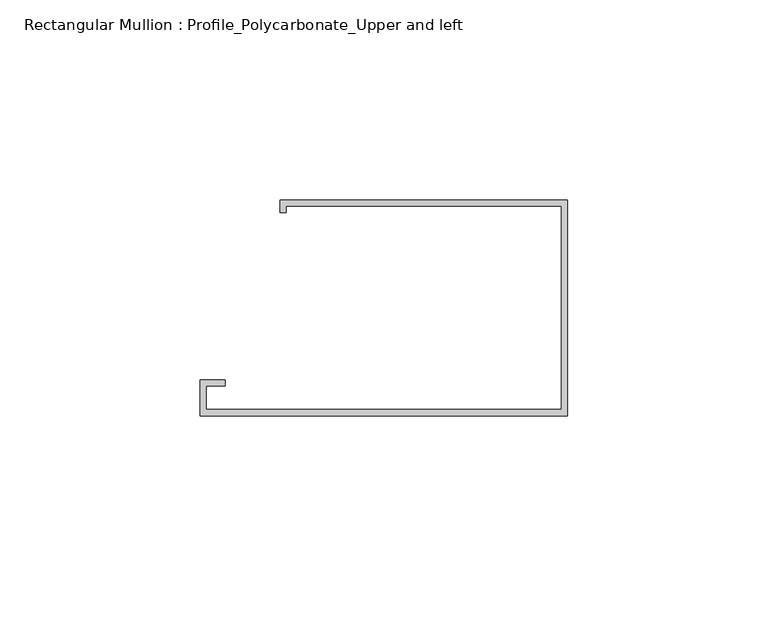
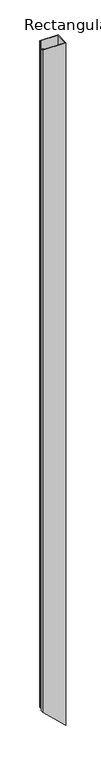
"""IFC4 building model written with IfcOpenShell, lengths in millimetres: member geometry, Rectangular Mullion : Profile_Polycarbonate_Upper and left."""

from ifc_helpers import new_model, si_unit, origin, place, context, project, spatial, faceted_brep, source, transform, mapped, element, save


def rectangular_mullion_profile_polycarbonate_upper_and_left_c928ab11(model_context):
    return source(origin(), model_context, "Body", "Brep", [
        faceted_brep([(0.0, -28.984575, 0.0), (0.0, 25.015825, 0.0), (-71.9836, 25.015825, 0.0), (-71.9836, 21.840825, 0.0), (-70.3961, 21.840825, 0.0), (-70.3961, 23.428325, 0.0), (-1.5875, 23.428325, 0.0), (-1.5875, -27.397075, 0.0), (-90.4113, -27.397075, 0.0), (-90.4113, -21.580475, 0.0), (-85.6488, -21.580475, 0.0), (-85.6488, -19.992975, 0.0), (-91.9988, -19.992975, 0.0), (-91.9988, -28.984575, 0.0), (0.0, -28.984575, -2875.2880888), (0.0, 25.015825, -2875.2880888), (-71.9836, 25.015825, -2806.2413468), (-71.9836, 21.840825, -2806.2413468), (-70.3961, 21.840825, -2807.7640784), (-70.3961, 23.428325, -2807.7640784), (-1.5875, 23.428325, -2873.7653572), (-1.5875, -27.397075, -2873.7653572), (-90.4113, -27.397075, -2788.5654783), (-90.4113, -21.580475, -2788.5654783), (-85.6488, -21.580475, -2793.1336732), (-85.6488, -19.992975, -2793.1336732), (-91.9988, -19.992975, -2787.0427467), (-91.9988, -28.984575, -2787.0427467)], [[[0, 1, 2, 3, 4, 5, 6, 7, 8, 9, 10, 11, 12, 13]], [[1, 0, 14, 15]], [[2, 1, 15, 16]], [[3, 2, 16, 17]], [[4, 3, 17, 18]], [[5, 4, 18, 19]], [[6, 5, 19, 20]], [[7, 6, 20, 21]], [[8, 7, 21, 22]], [[9, 8, 22, 23]], [[10, 9, 23, 24]], [[11, 10, 24, 25]], [[12, 11, 25, 26]], [[13, 12, 26, 27]], [[0, 13, 27, 14]], [[14, 27, 26, 25, 24, 23, 22, 21, 20, 19, 18, 17, 16, 15]]]),
    ])


if __name__ == "__main__":
    model = new_model("IFC4")
    model_context = context("Model", 3, world=origin())
    ifc_project = project(units=[si_unit("LENGTHUNIT", "METRE", prefix="MILLI")], contexts=[model_context])
    site = spatial("IfcSite", under=ifc_project)
    building = spatial("IfcBuilding", under=site)
    placement = place(None, origin())
    rectangular_mullion_profile_polycarbonate_upper_and_left_shape = rectangular_mullion_profile_polycarbonate_upper_and_left_c928ab11(model_context)
    element("IfcMember", 1, ObjectType="Rectangular Mullion : Profile_Polycarbonate_Upper and left", at=placement, inside=building, context=model_context, shape_type="MappedRepresentation", body=[
        mapped(rectangular_mullion_profile_polycarbonate_upper_and_left_shape, transform((0.0, 0.0, 0.0), x_axis=(1.0, 0.0, 0.0), y_axis=(0.0, 1.0, 0.0), z_axis=(0.0, 0.0, 1.0))),
    ])
    save(model, "model.ifc")

# Revit data of these elements
# Type "Rectangular Mullion : Profile_Polycarbonate_Upper and left"
#   built-in parameter 1007322 = 0.177167 (stored number, unit not read)
#   built-in parameter 1007321 = 0.00520833 (stored number, unit not read)
#   built-in parameter 1007320 = 0 (stored number, unit not read)
